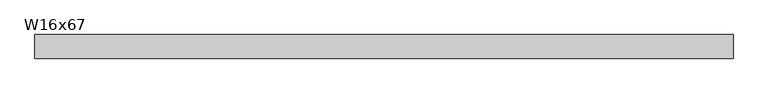
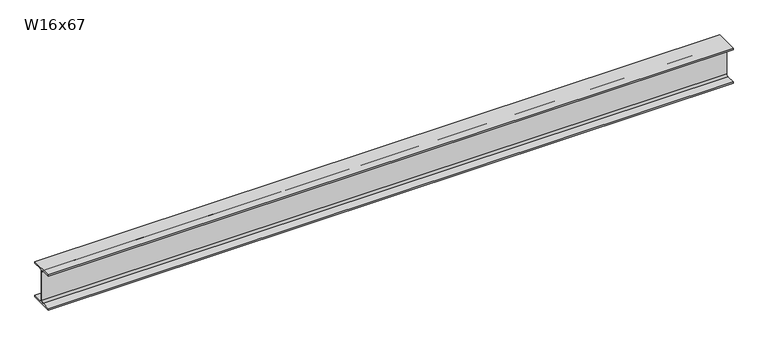
"""IFC4 building model written with IfcOpenShell, lengths in millimetres: beam geometry, RME W-Wide Flange : W16x67."""

from ifc_helpers import new_model, si_unit, point, frame, frame_2d, origin, place, context, project, spatial, polyline, circle_curve, trimmed, segment, composite_curve, outline, extrude, source, transform, mapped, element, save


def w16x67_0baf5f23(model_context):
    return source(origin(), model_context, "Body", "SweptSolid", [
        extrude(outline(composite_curve([segment(polyline([(129.54, -190.119), (129.54, -207.01), (-129.54, -207.01), (-129.54, -190.119), (-27.813, -190.119)]), True, "CONTINUOUS"), segment(trimmed(circle_curve(frame_2d((-27.813, -167.3225)), 22.7965), [point((-27.813, -190.119))], [point((-5.0165, -167.3225))], True, "CARTESIAN"), True, "CONTINUOUS"), segment(polyline([(-5.0165, -167.3225), (-5.0165, 167.3225)]), True, "CONTINUOUS"), segment(trimmed(circle_curve(frame_2d((-27.813, 167.3225)), 22.7965), [point((-5.0165, 167.3225))], [point((-27.813, 190.119))], True, "CARTESIAN"), True, "CONTINUOUS"), segment(polyline([(-27.813, 190.119), (-129.54, 190.119), (-129.54, 207.01), (129.54, 207.01), (129.54, 190.119), (27.813, 190.119)]), True, "CONTINUOUS"), segment(trimmed(circle_curve(frame_2d((27.813, 167.3225)), 22.7965), [point((27.813, 190.119))], [point((5.0165, 167.3225))], True, "CARTESIAN"), True, "CONTINUOUS"), segment(polyline([(5.0165, 167.3225), (5.0165, -167.3225)]), True, "CONTINUOUS"), segment(trimmed(circle_curve(frame_2d((27.813, -167.3225)), 22.7965), [point((5.0165, -167.3225))], [point((27.813, -190.119))], True, "CARTESIAN"), True, "CONTINUOUS"), segment(polyline([(27.813, -190.119), (129.54, -190.119)]), True, "CONTINUOUS")], self_intersect=False)), frame((-3822.7, 0.0, 0.0), z_axis=(1.0, 0.0, 0.0), x_axis=(0.0, 1.0, 0.0)), (0.0, 0.0, 1.0), 7645.4),
    ])


if __name__ == "__main__":
    model = new_model("IFC4")
    model_context = context("Model", 3, world=origin())
    ifc_project = project(units=[si_unit("LENGTHUNIT", "METRE", prefix="MILLI")], contexts=[model_context])
    site = spatial("IfcSite", under=ifc_project)
    building = spatial("IfcBuilding", under=site)
    placement = place(None, origin())
    w16x67_shape = w16x67_0baf5f23(model_context)
    element("IfcBeam", 1, ObjectType="RME W-Wide Flange : W16x67", at=placement, inside=building, context=model_context, shape_type="MappedRepresentation", body=[
        mapped(w16x67_shape, transform((0.0, 0.0, 0.0), x_axis=(1.0, 0.0, 0.0), y_axis=(0.0, 1.0, 0.0), z_axis=(0.0, 0.0, 1.0))),
    ])
    save(model, "model.ifc")

# Revit data of these elements
# Type "RME W-Wide Flange : W16x67"
#   WELD P [instance default] = ""
#   WELD LE [instance default] = ""
#   WELD D [instance default] = ""
#   TOP SECTION SIZE [instance default] = ""
#   TOP SECTION LENGTH [instance default] = ""
#   REMARKS [instance default] = ""
#   REINF TYPE [instance default] = ""
#   Nominal Size = "W24"
#   End Bearing Capacity [instance default] = ""
#   BOT SECTION SIZE [instance default] = ""
#   BOT SECTION LENGTH [instance default] = ""
#   Assembly Code = "B10"
#   W = 67
#   Start Extension Calculation [instance default] = 10' - 0"
#   Start Extension [instance default] = -0' - 0 1/2"
#   End Extension Calculation [instance default] = 10' - 0"
#   End Extension [instance default] = -0' - 0 1/2"
#   Length [instance default] = 5' - 0"
#   bf = 0' - 10.2"
#   d = 1' - 4.3"
#   k = 0' - 1 9/16"
#   k2 = 0' - 0.8975"
#   tf = 0' - 0.665"
#   tw = 0' - 0.395"
#   A = 0.136806 SF
#   Structural Material [instance default] = Metal - Steel - ASTM A992
# Element 1 (IfcBeam, "RME W-Wide Flange : W16x67")
#   Length = 25' - 10"
#   Materials on its faces: "Metal - Steel - ASTM A992"
# Materials
#   "Metal - Steel - ASTM A992": class "Metal", colour RGB 255 128 0, transparency 0
